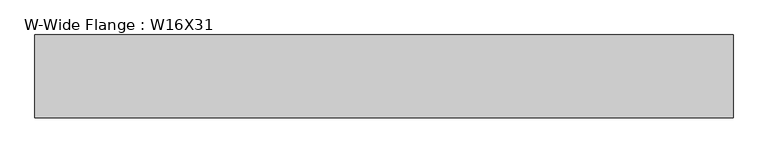
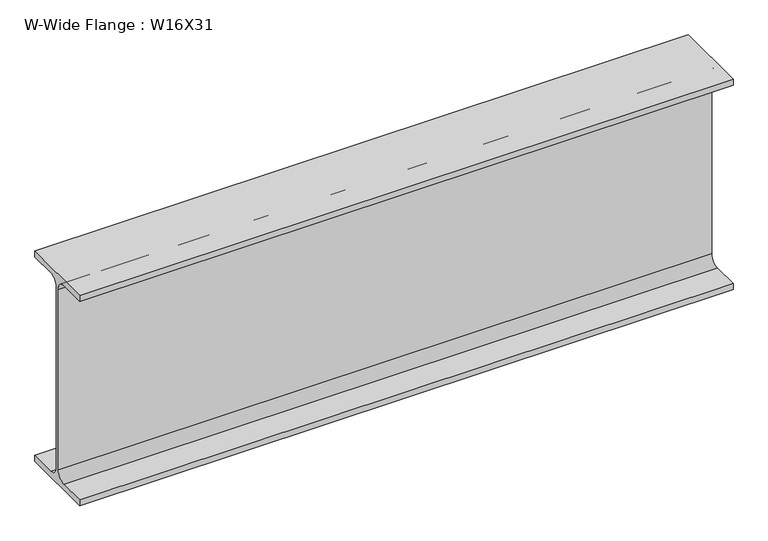
"""IFC4 building model written with IfcOpenShell, lengths in millimetres: beam geometry, W-Wide Flange : W16X31."""

from ifc_helpers import new_model, si_unit, point, frame, frame_2d, origin, place, context, project, spatial, polyline, circle_curve, trimmed, segment, composite_curve, outline, extrude, source, transform, mapped, element, save


def w_wide_flange_w16x31_b5bae09e(model_context):
    return source(origin(), model_context, "Body", "SweptSolid", [
        extrude(outline(composite_curve([segment(polyline([(70.231, -190.754), (70.231, -201.93), (-70.231, -201.93), (-70.231, -190.754), (-20.8915, -190.754)]), True, "CONTINUOUS"), segment(trimmed(circle_curve(frame_2d((-20.8915, -173.355)), 17.399), [point((-20.8915, -190.754))], [point((-3.4925, -173.355))], True, "CARTESIAN"), True, "CONTINUOUS"), segment(polyline([(-3.4925, -173.355), (-3.4925, 173.355)]), True, "CONTINUOUS"), segment(trimmed(circle_curve(frame_2d((-20.8915, 173.355)), 17.399), [point((-3.4925, 173.355))], [point((-20.8915, 190.754))], True, "CARTESIAN"), True, "CONTINUOUS"), segment(polyline([(-20.8915, 190.754), (-70.231, 190.754), (-70.231, 201.93), (70.231, 201.93), (70.231, 190.754), (20.8915, 190.754)]), True, "CONTINUOUS"), segment(trimmed(circle_curve(frame_2d((20.8915, 173.355)), 17.399), [point((20.8915, 190.754))], [point((3.4925, 173.355))], True, "CARTESIAN"), True, "CONTINUOUS"), segment(polyline([(3.4925, 173.355), (3.4925, -173.355)]), True, "CONTINUOUS"), segment(trimmed(circle_curve(frame_2d((20.8915, -173.355)), 17.399), [point((3.4925, -173.355))], [point((20.8915, -190.754))], True, "CARTESIAN"), True, "CONTINUOUS"), segment(polyline([(20.8915, -190.754), (70.231, -190.754)]), True, "CONTINUOUS")], self_intersect=False)), frame((-509.2048706, 0.0, 0.0), z_axis=(1.0, 0.0, 0.0), x_axis=(0.0, 1.0, 0.0)), (0.0, 0.0, 1.0), 1185.9337831),
    ])


if __name__ == "__main__":
    model = new_model("IFC4")
    model_context = context("Model", 3, world=origin())
    ifc_project = project(units=[si_unit("LENGTHUNIT", "METRE", prefix="MILLI")], contexts=[model_context])
    site = spatial("IfcSite", under=ifc_project)
    building = spatial("IfcBuilding", under=site)
    placement = place(None, origin())
    w_wide_flange_w16x31_shape = w_wide_flange_w16x31_b5bae09e(model_context)
    element("IfcBeam", 1, ObjectType="W-Wide Flange : W16X31", at=placement, inside=building, context=model_context, shape_type="MappedRepresentation", body=[
        mapped(w_wide_flange_w16x31_shape, transform((0.0, 0.0, 0.0), x_axis=(1.0, 0.0, 0.0), y_axis=(0.0, 1.0, 0.0), z_axis=(0.0, 0.0, 1.0))),
    ])
    save(model, "model.ifc")

# Revit data of these elements
# Type "W-Wide Flange : W16X31"
#   Assembly Code = "B10"
#   W = 31
#   Start Extension Calculation [instance default] = 10' - 0"
#   Start Extension [instance default] = -0' - 0 1/2"
#   End Extension Calculation [instance default] = 10' - 0"
#   End Extension [instance default] = -0' - 0 1/2"
#   Length [instance default] = 5' - 0"
#   bf = 0' - 5.53"
#   d = 1' - 3.9"
#   k = 0' - 1 1/8"
#   k2 = 0' - 0.685"
#   tf = 0' - 0.44"
#   tw = 0' - 0.275"
#   A = 0.0634028 SF
#   Beam Material [instance default] = Metal - Steel - ASTM A992
# Element 1 (IfcBeam, "W-Wide Flange : W16X31")
#   Materials on its faces: "Metal - Steel - ASTM A992"
# Materials
#   "Metal - Steel - ASTM A992": class "Metal", colour RGB 128 0 0, transparency 0
